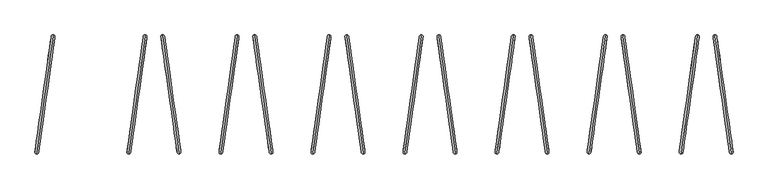
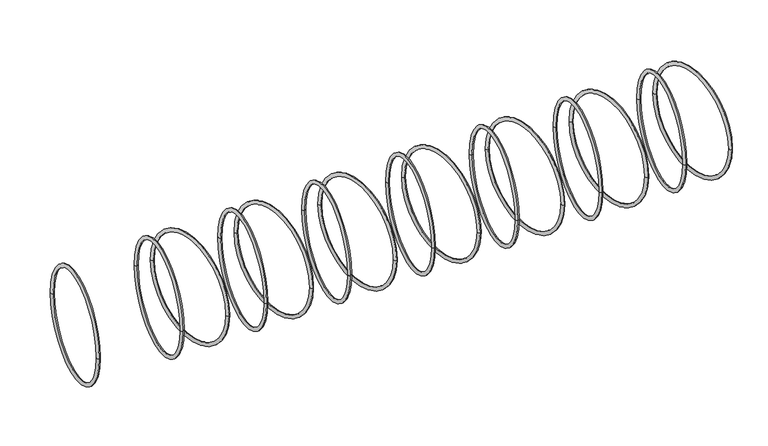
"""IFC4 building model written with IfcOpenShell, lengths in millimetres: geographic element geometry, NLRS_90_SI_WPB_fietsenrek staal_gen_bf : fietsenrek 5500mm 14 plaatsen."""

from ifc_helpers import new_model, si_unit, point, frame, origin, place, context, project, spatial, circle_curve, ellipse_curve, trimmed, source, transform, mapped, element, save
from ifc_brep_helpers import revolved_surface, advanced_brep


def geographic_element_08e1790a(model_context):
    return source(origin(), model_context, "Body", "AdvancedBrep", [
        advanced_brep(
        [(2160.5888305, -21.9255981, 304.7993564), (2092.0982681, -509.2612714, 304.7993564), (2089.8888952, -524.981777, 304.7993564), (2162.7982034, -6.2050925, 304.7993564)],
        [
            (0, 1, circle_curve(frame((2126.3435493, -265.5934347, 304.7993564), z_axis=(0.990268068741571, -0.13917310096006058, 0.0), x_axis=(-0.13917310096006058, -0.990268068741571, 0.0)), 246.0625)),
            (1, 2, circle_curve(frame((2090.9935817, -517.1215242, 304.7993564), z_axis=(0.0, 0.0, 1.0), x_axis=(0.13917310096006055, 0.990268068741571, 0.0)), 7.9375)),
            (2, 3, circle_curve(frame((2126.3435493, -265.5934347, 304.7993564), z_axis=(-0.990268068741571, 0.13917310096006058, 0.0), x_axis=(-0.13917310096006058, -0.990268068741571, 0.0)), 261.9375)),
            (3, 0, circle_curve(frame((2161.6935169, -14.0653453, 304.7993564), z_axis=(0.0, 0.0, 1.0), x_axis=(-0.1391731009600606, -0.990268068741571, 0.0)), 7.9375)),
            (2, 1, circle_curve(frame((2090.9935817, -517.1215242, 304.7993564), z_axis=(0.0, 0.0, 1.0), x_axis=(0.13917310096006055, 0.990268068741571, 0.0)), 7.9375)),
            (0, 3, circle_curve(frame((2161.6935169, -14.0653453, 304.7993564), z_axis=(0.0, 0.0, 1.0), x_axis=(-0.1391731009600606, -0.990268068741571, 0.0)), 7.9375)),
            (1, 0, circle_curve(frame((2126.3435493, -265.5934347, 304.7993564), z_axis=(0.990268068741571, -0.13917310096006058, 0.0), x_axis=(0.13917310096006058, 0.990268068741571, 0.0)), 246.0625)),
            (3, 2, circle_curve(frame((2126.3435493, -265.5934347, 304.7993564), z_axis=(-0.990268068741571, 0.13917310096006058, 0.0), x_axis=(0.13917310096006058, 0.990268068741571, 0.0)), 261.9375)),
        ],
        [
            revolved_surface(trimmed(ellipse_curve(frame((2090.9935817, -517.1215242, 304.7993564), z_axis=(0.0, 0.0, -1.0), x_axis=(0.13917310096006055, 0.990268068741571, 0.0)), 7.9375, 7.9375), [point((2089.8888952, -524.981777, 304.7993564))], [point((2092.0982681, -509.2612714, 304.7993564))], True, "CARTESIAN"), (2314.9896164, -292.1059105, 304.7993564), (-0.990268068741571, 0.13917310096006058, 0.0)),
            revolved_surface(trimmed(ellipse_curve(frame((2090.9935817, -517.1215242, 304.7993564), z_axis=(0.0, 0.0, -1.0), x_axis=(0.13917310096006055, 0.990268068741571, 0.0)), 7.9375, 7.9375), [point((2092.0982681, -509.2612714, 304.7993564))], [point((2089.8888952, -524.981777, 304.7993564))], True, "CARTESIAN"), (2314.9896164, -292.1059105, 304.7993564), (-0.990268068741571, 0.13917310096006058, 0.0)),
            revolved_surface(trimmed(ellipse_curve(frame((2161.6935169, -14.0653453, 304.7993564), z_axis=(0.0, 0.0, 1.0), x_axis=(-0.13917310096006055, -0.990268068741571, 0.0)), 7.9375, 7.9375), [point((2162.7982034, -6.2050925, 304.7993564))], [point((2160.5888305, -21.9255981, 304.7993564))], True, "CARTESIAN"), (2314.9896164, -292.1059105, 304.7993564), (-0.990268068741571, 0.13917310096006058, 0.0)),
            revolved_surface(trimmed(ellipse_curve(frame((2161.6935169, -14.0653453, 304.7993564), z_axis=(0.0, 0.0, 1.0), x_axis=(-0.13917310096006055, -0.990268068741571, 0.0)), 7.9375, 7.9375), [point((2160.5888305, -21.9255981, 304.7993564))], [point((2162.7982034, -6.2050925, 304.7993564))], True, "CARTESIAN"), (2314.9896164, -292.1059105, 304.7993564), (-0.990268068741571, 0.13917310096006058, 0.0)),
        ],
        [
            (0, [[1, 2, 3, 4]]),
            (1, [[-3, 5, -1, 6]]),
            (2, [[7, -4, 8, -2]]),
            (3, [[-8, -6, -7, -5]]),
        ],
    ),
        advanced_brep(
        [(2239.4111695, -21.9255981, 304.7993564), (2307.9017319, -509.2612714, 304.7993564), (2310.1111048, -524.981777, 304.7993564), (2237.2017966, -6.2050925, 304.7993564)],
        [
            (0, 1, circle_curve(frame((2273.6564507, -265.5934347, 304.7993564), z_axis=(0.9902680687415715, 0.1391731009600577, 0.0), x_axis=(0.1391731009600577, -0.9902680687415715, 0.0)), 246.0625)),
            (1, 2, circle_curve(frame((2309.0064183, -517.1215242, 304.7993564), z_axis=(0.0, 0.0, 1.0), x_axis=(-0.13917310096005775, 0.9902680687415715, 0.0)), 7.9375)),
            (2, 3, circle_curve(frame((2273.6564507, -265.5934347, 304.7993564), z_axis=(-0.9902680687415715, -0.1391731009600577, 0.0), x_axis=(0.1391731009600577, -0.9902680687415715, 0.0)), 261.9375)),
            (3, 0, circle_curve(frame((2238.3064831, -14.0653453, 304.7993564), z_axis=(0.0, 0.0, 1.0), x_axis=(0.13917310096005764, -0.9902680687415715, 0.0)), 7.9375)),
            (2, 1, circle_curve(frame((2309.0064183, -517.1215242, 304.7993564), z_axis=(0.0, 0.0, 1.0), x_axis=(-0.13917310096005775, 0.9902680687415715, 0.0)), 7.9375)),
            (0, 3, circle_curve(frame((2238.3064831, -14.0653453, 304.7993564), z_axis=(0.0, 0.0, 1.0), x_axis=(0.13917310096005764, -0.9902680687415715, 0.0)), 7.9375)),
            (1, 0, circle_curve(frame((2273.6564507, -265.5934347, 304.7993564), z_axis=(0.9902680687415715, 0.1391731009600577, 0.0), x_axis=(-0.1391731009600577, 0.9902680687415715, 0.0)), 246.0625)),
            (3, 2, circle_curve(frame((2273.6564507, -265.5934347, 304.7993564), z_axis=(-0.9902680687415715, -0.1391731009600577, 0.0), x_axis=(-0.1391731009600577, 0.9902680687415715, 0.0)), 261.9375)),
        ],
        [
            revolved_surface(trimmed(ellipse_curve(frame((2309.0064183, -517.1215242, 304.7993564), z_axis=(0.0, 0.0, -1.0), x_axis=(-0.13917310096005775, 0.9902680687415715, 0.0)), 7.9375, 7.9375), [point((2310.1111048, -524.981777, 304.7993564))], [point((2307.9017319, -509.2612714, 304.7993564))], True, "CARTESIAN"), (2085.0103836, -292.1059105, 304.7993564), (-0.9902680687415715, -0.1391731009600577, 0.0)),
            revolved_surface(trimmed(ellipse_curve(frame((2309.0064183, -517.1215242, 304.7993564), z_axis=(0.0, 0.0, -1.0), x_axis=(-0.13917310096005775, 0.9902680687415715, 0.0)), 7.9375, 7.9375), [point((2307.9017319, -509.2612714, 304.7993564))], [point((2310.1111048, -524.981777, 304.7993564))], True, "CARTESIAN"), (2085.0103836, -292.1059105, 304.7993564), (-0.9902680687415715, -0.1391731009600577, 0.0)),
            revolved_surface(trimmed(ellipse_curve(frame((2238.3064831, -14.0653453, 304.7993564), z_axis=(0.0, 0.0, 1.0), x_axis=(0.1391731009600577, -0.9902680687415715, 0.0)), 7.9375, 7.9375), [point((2237.2017966, -6.2050925, 304.7993564))], [point((2239.4111695, -21.9255981, 304.7993564))], True, "CARTESIAN"), (2085.0103836, -292.1059105, 304.7993564), (-0.9902680687415715, -0.1391731009600577, 0.0)),
            revolved_surface(trimmed(ellipse_curve(frame((2238.3064831, -14.0653453, 304.7993564), z_axis=(0.0, 0.0, 1.0), x_axis=(0.1391731009600577, -0.9902680687415715, 0.0)), 7.9375, 7.9375), [point((2239.4111695, -21.9255981, 304.7993564))], [point((2237.2017966, -6.2050925, 304.7993564))], True, "CARTESIAN"), (2085.0103836, -292.1059105, 304.7993564), (-0.9902680687415715, -0.1391731009600577, 0.0)),
        ],
        [
            (0, [[1, 2, 3, 4]]),
            (1, [[-3, 5, -1, 6]]),
            (2, [[7, -4, 8, -2]]),
            (3, [[-8, -6, -7, -5]]),
        ],
    ),
        advanced_brep(
        [(1760.5888305, -21.9255981, 304.7993564), (1692.0982681, -509.2612714, 304.7993564), (1689.8888952, -524.981777, 304.7993564), (1762.7982034, -6.2050925, 304.7993564)],
        [
            (0, 1, circle_curve(frame((1726.3435493, -265.5934347, 304.7993564), z_axis=(0.990268068741571, -0.13917310096006058, 0.0), x_axis=(-0.13917310096006058, -0.990268068741571, 0.0)), 246.0625)),
            (1, 2, circle_curve(frame((1690.9935817, -517.1215242, 304.7993564), z_axis=(0.0, 0.0, 1.0), x_axis=(0.13917310096006055, 0.990268068741571, 0.0)), 7.9375)),
            (2, 3, circle_curve(frame((1726.3435493, -265.5934347, 304.7993564), z_axis=(-0.990268068741571, 0.13917310096006058, 0.0), x_axis=(-0.13917310096006058, -0.990268068741571, 0.0)), 261.9375)),
            (3, 0, circle_curve(frame((1761.6935169, -14.0653453, 304.7993564), z_axis=(0.0, 0.0, 1.0), x_axis=(-0.1391731009600606, -0.990268068741571, 0.0)), 7.9375)),
            (2, 1, circle_curve(frame((1690.9935817, -517.1215242, 304.7993564), z_axis=(0.0, 0.0, 1.0), x_axis=(0.13917310096006055, 0.990268068741571, 0.0)), 7.9375)),
            (0, 3, circle_curve(frame((1761.6935169, -14.0653453, 304.7993564), z_axis=(0.0, 0.0, 1.0), x_axis=(-0.1391731009600606, -0.990268068741571, 0.0)), 7.9375)),
            (1, 0, circle_curve(frame((1726.3435493, -265.5934347, 304.7993564), z_axis=(0.990268068741571, -0.13917310096006058, 0.0), x_axis=(0.13917310096006058, 0.990268068741571, 0.0)), 246.0625)),
            (3, 2, circle_curve(frame((1726.3435493, -265.5934347, 304.7993564), z_axis=(-0.990268068741571, 0.13917310096006058, 0.0), x_axis=(0.13917310096006058, 0.990268068741571, 0.0)), 261.9375)),
        ],
        [
            revolved_surface(trimmed(ellipse_curve(frame((1690.9935817, -517.1215242, 304.7993564), z_axis=(0.0, 0.0, -1.0), x_axis=(0.13917310096006055, 0.990268068741571, 0.0)), 7.9375, 7.9375), [point((1689.8888952, -524.981777, 304.7993564))], [point((1692.0982681, -509.2612714, 304.7993564))], True, "CARTESIAN"), (1914.9896164, -292.1059105, 304.7993564), (-0.990268068741571, 0.13917310096006058, 0.0)),
            revolved_surface(trimmed(ellipse_curve(frame((1690.9935817, -517.1215242, 304.7993564), z_axis=(0.0, 0.0, -1.0), x_axis=(0.13917310096006055, 0.990268068741571, 0.0)), 7.9375, 7.9375), [point((1692.0982681, -509.2612714, 304.7993564))], [point((1689.8888952, -524.981777, 304.7993564))], True, "CARTESIAN"), (1914.9896164, -292.1059105, 304.7993564), (-0.990268068741571, 0.13917310096006058, 0.0)),
            revolved_surface(trimmed(ellipse_curve(frame((1761.6935169, -14.0653453, 304.7993564), z_axis=(0.0, 0.0, 1.0), x_axis=(-0.13917310096006055, -0.990268068741571, 0.0)), 7.9375, 7.9375), [point((1762.7982034, -6.2050925, 304.7993564))], [point((1760.5888305, -21.9255981, 304.7993564))], True, "CARTESIAN"), (1914.9896164, -292.1059105, 304.7993564), (-0.990268068741571, 0.13917310096006058, 0.0)),
            revolved_surface(trimmed(ellipse_curve(frame((1761.6935169, -14.0653453, 304.7993564), z_axis=(0.0, 0.0, 1.0), x_axis=(-0.13917310096006055, -0.990268068741571, 0.0)), 7.9375, 7.9375), [point((1760.5888305, -21.9255981, 304.7993564))], [point((1762.7982034, -6.2050925, 304.7993564))], True, "CARTESIAN"), (1914.9896164, -292.1059105, 304.7993564), (-0.990268068741571, 0.13917310096006058, 0.0)),
        ],
        [
            (0, [[1, 2, 3, 4]]),
            (1, [[-3, 5, -1, 6]]),
            (2, [[7, -4, 8, -2]]),
            (3, [[-8, -6, -7, -5]]),
        ],
    ),
        advanced_brep(
        [(1839.4111695, -21.9255981, 304.7993564), (1907.9017319, -509.2612714, 304.7993564), (1910.1111048, -524.981777, 304.7993564), (1837.2017966, -6.2050925, 304.7993564)],
        [
            (0, 1, circle_curve(frame((1873.6564507, -265.5934347, 304.7993564), z_axis=(0.9902680687415715, 0.1391731009600577, 0.0), x_axis=(0.1391731009600577, -0.9902680687415715, 0.0)), 246.0625)),
            (1, 2, circle_curve(frame((1909.0064183, -517.1215242, 304.7993564), z_axis=(0.0, 0.0, 1.0), x_axis=(-0.13917310096005775, 0.9902680687415715, 0.0)), 7.9375)),
            (2, 3, circle_curve(frame((1873.6564507, -265.5934347, 304.7993564), z_axis=(-0.9902680687415715, -0.1391731009600577, 0.0), x_axis=(0.1391731009600577, -0.9902680687415715, 0.0)), 261.9375)),
            (3, 0, circle_curve(frame((1838.3064831, -14.0653453, 304.7993564), z_axis=(0.0, 0.0, 1.0), x_axis=(0.13917310096005764, -0.9902680687415715, 0.0)), 7.9375)),
            (2, 1, circle_curve(frame((1909.0064183, -517.1215242, 304.7993564), z_axis=(0.0, 0.0, 1.0), x_axis=(-0.13917310096005775, 0.9902680687415715, 0.0)), 7.9375)),
            (0, 3, circle_curve(frame((1838.3064831, -14.0653453, 304.7993564), z_axis=(0.0, 0.0, 1.0), x_axis=(0.13917310096005764, -0.9902680687415715, 0.0)), 7.9375)),
            (1, 0, circle_curve(frame((1873.6564507, -265.5934347, 304.7993564), z_axis=(0.9902680687415715, 0.1391731009600577, 0.0), x_axis=(-0.1391731009600577, 0.9902680687415715, 0.0)), 246.0625)),
            (3, 2, circle_curve(frame((1873.6564507, -265.5934347, 304.7993564), z_axis=(-0.9902680687415715, -0.1391731009600577, 0.0), x_axis=(-0.1391731009600577, 0.9902680687415715, 0.0)), 261.9375)),
        ],
        [
            revolved_surface(trimmed(ellipse_curve(frame((1909.0064183, -517.1215242, 304.7993564), z_axis=(0.0, 0.0, -1.0), x_axis=(-0.13917310096005775, 0.9902680687415715, 0.0)), 7.9375, 7.9375), [point((1910.1111048, -524.981777, 304.7993564))], [point((1907.9017319, -509.2612714, 304.7993564))], True, "CARTESIAN"), (1685.0103836, -292.1059105, 304.7993564), (-0.9902680687415715, -0.1391731009600577, 0.0)),
            revolved_surface(trimmed(ellipse_curve(frame((1909.0064183, -517.1215242, 304.7993564), z_axis=(0.0, 0.0, -1.0), x_axis=(-0.13917310096005775, 0.9902680687415715, 0.0)), 7.9375, 7.9375), [point((1907.9017319, -509.2612714, 304.7993564))], [point((1910.1111048, -524.981777, 304.7993564))], True, "CARTESIAN"), (1685.0103836, -292.1059105, 304.7993564), (-0.9902680687415715, -0.1391731009600577, 0.0)),
            revolved_surface(trimmed(ellipse_curve(frame((1838.3064831, -14.0653453, 304.7993564), z_axis=(0.0, 0.0, 1.0), x_axis=(0.1391731009600577, -0.9902680687415715, 0.0)), 7.9375, 7.9375), [point((1837.2017966, -6.2050925, 304.7993564))], [point((1839.4111695, -21.9255981, 304.7993564))], True, "CARTESIAN"), (1685.0103836, -292.1059105, 304.7993564), (-0.9902680687415715, -0.1391731009600577, 0.0)),
            revolved_surface(trimmed(ellipse_curve(frame((1838.3064831, -14.0653453, 304.7993564), z_axis=(0.0, 0.0, 1.0), x_axis=(0.1391731009600577, -0.9902680687415715, 0.0)), 7.9375, 7.9375), [point((1839.4111695, -21.9255981, 304.7993564))], [point((1837.2017966, -6.2050925, 304.7993564))], True, "CARTESIAN"), (1685.0103836, -292.1059105, 304.7993564), (-0.9902680687415715, -0.1391731009600577, 0.0)),
        ],
        [
            (0, [[1, 2, 3, 4]]),
            (1, [[-3, 5, -1, 6]]),
            (2, [[7, -4, 8, -2]]),
            (3, [[-8, -6, -7, -5]]),
        ],
    ),
        advanced_brep(
        [(1360.5888305, -21.9255981, 304.7993564), (1292.0982681, -509.2612714, 304.7993564), (1289.8888952, -524.981777, 304.7993564), (1362.7982034, -6.2050925, 304.7993564)],
        [
            (0, 1, circle_curve(frame((1326.3435493, -265.5934347, 304.7993564), z_axis=(0.990268068741571, -0.13917310096006058, 0.0), x_axis=(-0.13917310096006058, -0.990268068741571, 0.0)), 246.0625)),
            (1, 2, circle_curve(frame((1290.9935817, -517.1215242, 304.7993564), z_axis=(0.0, 0.0, 1.0), x_axis=(0.13917310096006055, 0.990268068741571, 0.0)), 7.9375)),
            (2, 3, circle_curve(frame((1326.3435493, -265.5934347, 304.7993564), z_axis=(-0.990268068741571, 0.13917310096006058, 0.0), x_axis=(-0.13917310096006058, -0.990268068741571, 0.0)), 261.9375)),
            (3, 0, circle_curve(frame((1361.6935169, -14.0653453, 304.7993564), z_axis=(0.0, 0.0, 1.0), x_axis=(-0.1391731009600606, -0.990268068741571, 0.0)), 7.9375)),
            (2, 1, circle_curve(frame((1290.9935817, -517.1215242, 304.7993564), z_axis=(0.0, 0.0, 1.0), x_axis=(0.13917310096006055, 0.990268068741571, 0.0)), 7.9375)),
            (0, 3, circle_curve(frame((1361.6935169, -14.0653453, 304.7993564), z_axis=(0.0, 0.0, 1.0), x_axis=(-0.1391731009600606, -0.990268068741571, 0.0)), 7.9375)),
            (1, 0, circle_curve(frame((1326.3435493, -265.5934347, 304.7993564), z_axis=(0.990268068741571, -0.13917310096006058, 0.0), x_axis=(0.13917310096006058, 0.990268068741571, 0.0)), 246.0625)),
            (3, 2, circle_curve(frame((1326.3435493, -265.5934347, 304.7993564), z_axis=(-0.990268068741571, 0.13917310096006058, 0.0), x_axis=(0.13917310096006058, 0.990268068741571, 0.0)), 261.9375)),
        ],
        [
            revolved_surface(trimmed(ellipse_curve(frame((1290.9935817, -517.1215242, 304.7993564), z_axis=(0.0, 0.0, -1.0), x_axis=(0.13917310096006055, 0.990268068741571, 0.0)), 7.9375, 7.9375), [point((1289.8888952, -524.981777, 304.7993564))], [point((1292.0982681, -509.2612714, 304.7993564))], True, "CARTESIAN"), (1514.9896164, -292.1059105, 304.7993564), (-0.990268068741571, 0.13917310096006058, 0.0)),
            revolved_surface(trimmed(ellipse_curve(frame((1290.9935817, -517.1215242, 304.7993564), z_axis=(0.0, 0.0, -1.0), x_axis=(0.13917310096006055, 0.990268068741571, 0.0)), 7.9375, 7.9375), [point((1292.0982681, -509.2612714, 304.7993564))], [point((1289.8888952, -524.981777, 304.7993564))], True, "CARTESIAN"), (1514.9896164, -292.1059105, 304.7993564), (-0.990268068741571, 0.13917310096006058, 0.0)),
            revolved_surface(trimmed(ellipse_curve(frame((1361.6935169, -14.0653453, 304.7993564), z_axis=(0.0, 0.0, 1.0), x_axis=(-0.13917310096006055, -0.990268068741571, 0.0)), 7.9375, 7.9375), [point((1362.7982034, -6.2050925, 304.7993564))], [point((1360.5888305, -21.9255981, 304.7993564))], True, "CARTESIAN"), (1514.9896164, -292.1059105, 304.7993564), (-0.990268068741571, 0.13917310096006058, 0.0)),
            revolved_surface(trimmed(ellipse_curve(frame((1361.6935169, -14.0653453, 304.7993564), z_axis=(0.0, 0.0, 1.0), x_axis=(-0.13917310096006055, -0.990268068741571, 0.0)), 7.9375, 7.9375), [point((1360.5888305, -21.9255981, 304.7993564))], [point((1362.7982034, -6.2050925, 304.7993564))], True, "CARTESIAN"), (1514.9896164, -292.1059105, 304.7993564), (-0.990268068741571, 0.13917310096006058, 0.0)),
        ],
        [
            (0, [[1, 2, 3, 4]]),
            (1, [[-3, 5, -1, 6]]),
            (2, [[7, -4, 8, -2]]),
            (3, [[-8, -6, -7, -5]]),
        ],
    ),
        advanced_brep(
        [(1439.4111695, -21.9255981, 304.7993564), (1507.9017319, -509.2612714, 304.7993564), (1510.1111048, -524.981777, 304.7993564), (1437.2017966, -6.2050925, 304.7993564)],
        [
            (0, 1, circle_curve(frame((1473.6564507, -265.5934347, 304.7993564), z_axis=(0.9902680687415715, 0.1391731009600577, 0.0), x_axis=(0.1391731009600577, -0.9902680687415715, 0.0)), 246.0625)),
            (1, 2, circle_curve(frame((1509.0064183, -517.1215242, 304.7993564), z_axis=(0.0, 0.0, 1.0), x_axis=(-0.13917310096005775, 0.9902680687415715, 0.0)), 7.9375)),
            (2, 3, circle_curve(frame((1473.6564507, -265.5934347, 304.7993564), z_axis=(-0.9902680687415715, -0.1391731009600577, 0.0), x_axis=(0.1391731009600577, -0.9902680687415715, 0.0)), 261.9375)),
            (3, 0, circle_curve(frame((1438.3064831, -14.0653453, 304.7993564), z_axis=(0.0, 0.0, 1.0), x_axis=(0.13917310096005764, -0.9902680687415715, 0.0)), 7.9375)),
            (2, 1, circle_curve(frame((1509.0064183, -517.1215242, 304.7993564), z_axis=(0.0, 0.0, 1.0), x_axis=(-0.13917310096005775, 0.9902680687415715, 0.0)), 7.9375)),
            (0, 3, circle_curve(frame((1438.3064831, -14.0653453, 304.7993564), z_axis=(0.0, 0.0, 1.0), x_axis=(0.13917310096005764, -0.9902680687415715, 0.0)), 7.9375)),
            (1, 0, circle_curve(frame((1473.6564507, -265.5934347, 304.7993564), z_axis=(0.9902680687415715, 0.1391731009600577, 0.0), x_axis=(-0.1391731009600577, 0.9902680687415715, 0.0)), 246.0625)),
            (3, 2, circle_curve(frame((1473.6564507, -265.5934347, 304.7993564), z_axis=(-0.9902680687415715, -0.1391731009600577, 0.0), x_axis=(-0.1391731009600577, 0.9902680687415715, 0.0)), 261.9375)),
        ],
        [
            revolved_surface(trimmed(ellipse_curve(frame((1509.0064183, -517.1215242, 304.7993564), z_axis=(0.0, 0.0, -1.0), x_axis=(-0.13917310096005775, 0.9902680687415715, 0.0)), 7.9375, 7.9375), [point((1510.1111048, -524.981777, 304.7993564))], [point((1507.9017319, -509.2612714, 304.7993564))], True, "CARTESIAN"), (1285.0103836, -292.1059105, 304.7993564), (-0.9902680687415715, -0.1391731009600577, 0.0)),
            revolved_surface(trimmed(ellipse_curve(frame((1509.0064183, -517.1215242, 304.7993564), z_axis=(0.0, 0.0, -1.0), x_axis=(-0.13917310096005775, 0.9902680687415715, 0.0)), 7.9375, 7.9375), [point((1507.9017319, -509.2612714, 304.7993564))], [point((1510.1111048, -524.981777, 304.7993564))], True, "CARTESIAN"), (1285.0103836, -292.1059105, 304.7993564), (-0.9902680687415715, -0.1391731009600577, 0.0)),
            revolved_surface(trimmed(ellipse_curve(frame((1438.3064831, -14.0653453, 304.7993564), z_axis=(0.0, 0.0, 1.0), x_axis=(0.1391731009600577, -0.9902680687415715, 0.0)), 7.9375, 7.9375), [point((1437.2017966, -6.2050925, 304.7993564))], [point((1439.4111695, -21.9255981, 304.7993564))], True, "CARTESIAN"), (1285.0103836, -292.1059105, 304.7993564), (-0.9902680687415715, -0.1391731009600577, 0.0)),
            revolved_surface(trimmed(ellipse_curve(frame((1438.3064831, -14.0653453, 304.7993564), z_axis=(0.0, 0.0, 1.0), x_axis=(0.1391731009600577, -0.9902680687415715, 0.0)), 7.9375, 7.9375), [point((1439.4111695, -21.9255981, 304.7993564))], [point((1437.2017966, -6.2050925, 304.7993564))], True, "CARTESIAN"), (1285.0103836, -292.1059105, 304.7993564), (-0.9902680687415715, -0.1391731009600577, 0.0)),
        ],
        [
            (0, [[1, 2, 3, 4]]),
            (1, [[-3, 5, -1, 6]]),
            (2, [[7, -4, 8, -2]]),
            (3, [[-8, -6, -7, -5]]),
        ],
    ),
        advanced_brep(
        [(960.5888305, -21.9255981, 304.7993564), (892.0982681, -509.2612714, 304.7993564), (889.8888952, -524.981777, 304.7993564), (962.7982034, -6.2050925, 304.7993564)],
        [
            (0, 1, circle_curve(frame((926.3435493, -265.5934347, 304.7993564), z_axis=(0.990268068741571, -0.13917310096006058, 0.0), x_axis=(-0.13917310096006058, -0.990268068741571, 0.0)), 246.0625)),
            (1, 2, circle_curve(frame((890.9935817, -517.1215242, 304.7993564), z_axis=(0.0, 0.0, 1.0), x_axis=(0.13917310096006055, 0.990268068741571, 0.0)), 7.9375)),
            (2, 3, circle_curve(frame((926.3435493, -265.5934347, 304.7993564), z_axis=(-0.990268068741571, 0.13917310096006058, 0.0), x_axis=(-0.13917310096006058, -0.990268068741571, 0.0)), 261.9375)),
            (3, 0, circle_curve(frame((961.6935169, -14.0653453, 304.7993564), z_axis=(0.0, 0.0, 1.0), x_axis=(-0.1391731009600606, -0.990268068741571, 0.0)), 7.9375)),
            (2, 1, circle_curve(frame((890.9935817, -517.1215242, 304.7993564), z_axis=(0.0, 0.0, 1.0), x_axis=(0.13917310096006055, 0.990268068741571, 0.0)), 7.9375)),
            (0, 3, circle_curve(frame((961.6935169, -14.0653453, 304.7993564), z_axis=(0.0, 0.0, 1.0), x_axis=(-0.1391731009600606, -0.990268068741571, 0.0)), 7.9375)),
            (1, 0, circle_curve(frame((926.3435493, -265.5934347, 304.7993564), z_axis=(0.990268068741571, -0.13917310096006058, 0.0), x_axis=(0.13917310096006058, 0.990268068741571, 0.0)), 246.0625)),
            (3, 2, circle_curve(frame((926.3435493, -265.5934347, 304.7993564), z_axis=(-0.990268068741571, 0.13917310096006058, 0.0), x_axis=(0.13917310096006058, 0.990268068741571, 0.0)), 261.9375)),
        ],
        [
            revolved_surface(trimmed(ellipse_curve(frame((890.9935817, -517.1215242, 304.7993564), z_axis=(0.0, 0.0, -1.0), x_axis=(0.13917310096006055, 0.990268068741571, 0.0)), 7.9375, 7.9375), [point((889.8888952, -524.981777, 304.7993564))], [point((892.0982681, -509.2612714, 304.7993564))], True, "CARTESIAN"), (1114.9896164, -292.1059105, 304.7993564), (-0.990268068741571, 0.13917310096006058, 0.0)),
            revolved_surface(trimmed(ellipse_curve(frame((890.9935817, -517.1215242, 304.7993564), z_axis=(0.0, 0.0, -1.0), x_axis=(0.13917310096006055, 0.990268068741571, 0.0)), 7.9375, 7.9375), [point((892.0982681, -509.2612714, 304.7993564))], [point((889.8888952, -524.981777, 304.7993564))], True, "CARTESIAN"), (1114.9896164, -292.1059105, 304.7993564), (-0.990268068741571, 0.13917310096006058, 0.0)),
            revolved_surface(trimmed(ellipse_curve(frame((961.6935169, -14.0653453, 304.7993564), z_axis=(0.0, 0.0, 1.0), x_axis=(-0.13917310096006055, -0.990268068741571, 0.0)), 7.9375, 7.9375), [point((962.7982034, -6.2050925, 304.7993564))], [point((960.5888305, -21.9255981, 304.7993564))], True, "CARTESIAN"), (1114.9896164, -292.1059105, 304.7993564), (-0.990268068741571, 0.13917310096006058, 0.0)),
            revolved_surface(trimmed(ellipse_curve(frame((961.6935169, -14.0653453, 304.7993564), z_axis=(0.0, 0.0, 1.0), x_axis=(-0.13917310096006055, -0.990268068741571, 0.0)), 7.9375, 7.9375), [point((960.5888305, -21.9255981, 304.7993564))], [point((962.7982034, -6.2050925, 304.7993564))], True, "CARTESIAN"), (1114.9896164, -292.1059105, 304.7993564), (-0.990268068741571, 0.13917310096006058, 0.0)),
        ],
        [
            (0, [[1, 2, 3, 4]]),
            (1, [[-3, 5, -1, 6]]),
            (2, [[7, -4, 8, -2]]),
            (3, [[-8, -6, -7, -5]]),
        ],
    ),
        advanced_brep(
        [(1039.4111695, -21.9255981, 304.7993564), (1107.9017319, -509.2612714, 304.7993564), (1110.1111048, -524.981777, 304.7993564), (1037.2017966, -6.2050925, 304.7993564)],
        [
            (0, 1, circle_curve(frame((1073.6564507, -265.5934347, 304.7993564), z_axis=(0.9902680687415715, 0.1391731009600577, 0.0), x_axis=(0.1391731009600577, -0.9902680687415715, 0.0)), 246.0625)),
            (1, 2, circle_curve(frame((1109.0064183, -517.1215242, 304.7993564), z_axis=(0.0, 0.0, 1.0), x_axis=(-0.13917310096005775, 0.9902680687415715, 0.0)), 7.9375)),
            (2, 3, circle_curve(frame((1073.6564507, -265.5934347, 304.7993564), z_axis=(-0.9902680687415715, -0.1391731009600577, 0.0), x_axis=(0.1391731009600577, -0.9902680687415715, 0.0)), 261.9375)),
            (3, 0, circle_curve(frame((1038.3064831, -14.0653453, 304.7993564), z_axis=(0.0, 0.0, 1.0), x_axis=(0.13917310096005764, -0.9902680687415715, 0.0)), 7.9375)),
            (2, 1, circle_curve(frame((1109.0064183, -517.1215242, 304.7993564), z_axis=(0.0, 0.0, 1.0), x_axis=(-0.13917310096005775, 0.9902680687415715, 0.0)), 7.9375)),
            (0, 3, circle_curve(frame((1038.3064831, -14.0653453, 304.7993564), z_axis=(0.0, 0.0, 1.0), x_axis=(0.13917310096005764, -0.9902680687415715, 0.0)), 7.9375)),
            (1, 0, circle_curve(frame((1073.6564507, -265.5934347, 304.7993564), z_axis=(0.9902680687415715, 0.1391731009600577, 0.0), x_axis=(-0.1391731009600577, 0.9902680687415715, 0.0)), 246.0625)),
            (3, 2, circle_curve(frame((1073.6564507, -265.5934347, 304.7993564), z_axis=(-0.9902680687415715, -0.1391731009600577, 0.0), x_axis=(-0.1391731009600577, 0.9902680687415715, 0.0)), 261.9375)),
        ],
        [
            revolved_surface(trimmed(ellipse_curve(frame((1109.0064183, -517.1215242, 304.7993564), z_axis=(0.0, 0.0, -1.0), x_axis=(-0.13917310096005775, 0.9902680687415715, 0.0)), 7.9375, 7.9375), [point((1110.1111048, -524.981777, 304.7993564))], [point((1107.9017319, -509.2612714, 304.7993564))], True, "CARTESIAN"), (885.0103836, -292.1059105, 304.7993564), (-0.9902680687415715, -0.1391731009600577, 0.0)),
            revolved_surface(trimmed(ellipse_curve(frame((1109.0064183, -517.1215242, 304.7993564), z_axis=(0.0, 0.0, -1.0), x_axis=(-0.13917310096005775, 0.9902680687415715, 0.0)), 7.9375, 7.9375), [point((1107.9017319, -509.2612714, 304.7993564))], [point((1110.1111048, -524.981777, 304.7993564))], True, "CARTESIAN"), (885.0103836, -292.1059105, 304.7993564), (-0.9902680687415715, -0.1391731009600577, 0.0)),
            revolved_surface(trimmed(ellipse_curve(frame((1038.3064831, -14.0653453, 304.7993564), z_axis=(0.0, 0.0, 1.0), x_axis=(0.1391731009600577, -0.9902680687415715, 0.0)), 7.9375, 7.9375), [point((1037.2017966, -6.2050925, 304.7993564))], [point((1039.4111695, -21.9255981, 304.7993564))], True, "CARTESIAN"), (885.0103836, -292.1059105, 304.7993564), (-0.9902680687415715, -0.1391731009600577, 0.0)),
            revolved_surface(trimmed(ellipse_curve(frame((1038.3064831, -14.0653453, 304.7993564), z_axis=(0.0, 0.0, 1.0), x_axis=(0.1391731009600577, -0.9902680687415715, 0.0)), 7.9375, 7.9375), [point((1039.4111695, -21.9255981, 304.7993564))], [point((1037.2017966, -6.2050925, 304.7993564))], True, "CARTESIAN"), (885.0103836, -292.1059105, 304.7993564), (-0.9902680687415715, -0.1391731009600577, 0.0)),
        ],
        [
            (0, [[1, 2, 3, 4]]),
            (1, [[-3, 5, -1, 6]]),
            (2, [[7, -4, 8, -2]]),
            (3, [[-8, -6, -7, -5]]),
        ],
    ),
        advanced_brep(
        [(560.5888305, -21.9255981, 304.7993564), (492.0982681, -509.2612714, 304.7993564), (489.8888952, -524.981777, 304.7993564), (562.7982034, -6.2050925, 304.7993564)],
        [
            (0, 1, circle_curve(frame((526.3435493, -265.5934347, 304.7993564), z_axis=(0.990268068741571, -0.13917310096006058, 0.0), x_axis=(-0.13917310096006058, -0.990268068741571, 0.0)), 246.0625)),
            (1, 2, circle_curve(frame((490.9935817, -517.1215242, 304.7993564), z_axis=(0.0, 0.0, 1.0), x_axis=(0.13917310096006055, 0.990268068741571, 0.0)), 7.9375)),
            (2, 3, circle_curve(frame((526.3435493, -265.5934347, 304.7993564), z_axis=(-0.990268068741571, 0.13917310096006058, 0.0), x_axis=(-0.13917310096006058, -0.990268068741571, 0.0)), 261.9375)),
            (3, 0, circle_curve(frame((561.6935169, -14.0653453, 304.7993564), z_axis=(0.0, 0.0, 1.0), x_axis=(-0.1391731009600606, -0.990268068741571, 0.0)), 7.9375)),
            (2, 1, circle_curve(frame((490.9935817, -517.1215242, 304.7993564), z_axis=(0.0, 0.0, 1.0), x_axis=(0.13917310096006055, 0.990268068741571, 0.0)), 7.9375)),
            (0, 3, circle_curve(frame((561.6935169, -14.0653453, 304.7993564), z_axis=(0.0, 0.0, 1.0), x_axis=(-0.1391731009600606, -0.990268068741571, 0.0)), 7.9375)),
            (1, 0, circle_curve(frame((526.3435493, -265.5934347, 304.7993564), z_axis=(0.990268068741571, -0.13917310096006058, 0.0), x_axis=(0.13917310096006058, 0.990268068741571, 0.0)), 246.0625)),
            (3, 2, circle_curve(frame((526.3435493, -265.5934347, 304.7993564), z_axis=(-0.990268068741571, 0.13917310096006058, 0.0), x_axis=(0.13917310096006058, 0.990268068741571, 0.0)), 261.9375)),
        ],
        [
            revolved_surface(trimmed(ellipse_curve(frame((490.9935817, -517.1215242, 304.7993564), z_axis=(0.0, 0.0, -1.0), x_axis=(0.13917310096006055, 0.990268068741571, 0.0)), 7.9375, 7.9375), [point((489.8888952, -524.981777, 304.7993564))], [point((492.0982681, -509.2612714, 304.7993564))], True, "CARTESIAN"), (714.9896164, -292.1059105, 304.7993564), (-0.990268068741571, 0.13917310096006058, 0.0)),
            revolved_surface(trimmed(ellipse_curve(frame((490.9935817, -517.1215242, 304.7993564), z_axis=(0.0, 0.0, -1.0), x_axis=(0.13917310096006055, 0.990268068741571, 0.0)), 7.9375, 7.9375), [point((492.0982681, -509.2612714, 304.7993564))], [point((489.8888952, -524.981777, 304.7993564))], True, "CARTESIAN"), (714.9896164, -292.1059105, 304.7993564), (-0.990268068741571, 0.13917310096006058, 0.0)),
            revolved_surface(trimmed(ellipse_curve(frame((561.6935169, -14.0653453, 304.7993564), z_axis=(0.0, 0.0, 1.0), x_axis=(-0.13917310096006055, -0.990268068741571, 0.0)), 7.9375, 7.9375), [point((562.7982034, -6.2050925, 304.7993564))], [point((560.5888305, -21.9255981, 304.7993564))], True, "CARTESIAN"), (714.9896164, -292.1059105, 304.7993564), (-0.990268068741571, 0.13917310096006058, 0.0)),
            revolved_surface(trimmed(ellipse_curve(frame((561.6935169, -14.0653453, 304.7993564), z_axis=(0.0, 0.0, 1.0), x_axis=(-0.13917310096006055, -0.990268068741571, 0.0)), 7.9375, 7.9375), [point((560.5888305, -21.9255981, 304.7993564))], [point((562.7982034, -6.2050925, 304.7993564))], True, "CARTESIAN"), (714.9896164, -292.1059105, 304.7993564), (-0.990268068741571, 0.13917310096006058, 0.0)),
        ],
        [
            (0, [[1, 2, 3, 4]]),
            (1, [[-3, 5, -1, 6]]),
            (2, [[7, -4, 8, -2]]),
            (3, [[-8, -6, -7, -5]]),
        ],
    ),
        advanced_brep(
        [(639.4111695, -21.9255981, 304.7993564), (707.9017319, -509.2612714, 304.7993564), (710.1111048, -524.981777, 304.7993564), (637.2017966, -6.2050925, 304.7993564)],
        [
            (0, 1, circle_curve(frame((673.6564507, -265.5934347, 304.7993564), z_axis=(0.9902680687415715, 0.1391731009600577, 0.0), x_axis=(0.1391731009600577, -0.9902680687415715, 0.0)), 246.0625)),
            (1, 2, circle_curve(frame((709.0064183, -517.1215242, 304.7993564), z_axis=(0.0, 0.0, 1.0), x_axis=(-0.13917310096005775, 0.9902680687415715, 0.0)), 7.9375)),
            (2, 3, circle_curve(frame((673.6564507, -265.5934347, 304.7993564), z_axis=(-0.9902680687415715, -0.1391731009600577, 0.0), x_axis=(0.1391731009600577, -0.9902680687415715, 0.0)), 261.9375)),
            (3, 0, circle_curve(frame((638.3064831, -14.0653453, 304.7993564), z_axis=(0.0, 0.0, 1.0), x_axis=(0.13917310096005764, -0.9902680687415715, 0.0)), 7.9375)),
            (2, 1, circle_curve(frame((709.0064183, -517.1215242, 304.7993564), z_axis=(0.0, 0.0, 1.0), x_axis=(-0.13917310096005775, 0.9902680687415715, 0.0)), 7.9375)),
            (0, 3, circle_curve(frame((638.3064831, -14.0653453, 304.7993564), z_axis=(0.0, 0.0, 1.0), x_axis=(0.13917310096005764, -0.9902680687415715, 0.0)), 7.9375)),
            (1, 0, circle_curve(frame((673.6564507, -265.5934347, 304.7993564), z_axis=(0.9902680687415715, 0.1391731009600577, 0.0), x_axis=(-0.1391731009600577, 0.9902680687415715, 0.0)), 246.0625)),
            (3, 2, circle_curve(frame((673.6564507, -265.5934347, 304.7993564), z_axis=(-0.9902680687415715, -0.1391731009600577, 0.0), x_axis=(-0.1391731009600577, 0.9902680687415715, 0.0)), 261.9375)),
        ],
        [
            revolved_surface(trimmed(ellipse_curve(frame((709.0064183, -517.1215242, 304.7993564), z_axis=(0.0, 0.0, -1.0), x_axis=(-0.13917310096005775, 0.9902680687415715, 0.0)), 7.9375, 7.9375), [point((710.1111048, -524.981777, 304.7993564))], [point((707.9017319, -509.2612714, 304.7993564))], True, "CARTESIAN"), (485.0103836, -292.1059105, 304.7993564), (-0.9902680687415715, -0.1391731009600577, 0.0)),
            revolved_surface(trimmed(ellipse_curve(frame((709.0064183, -517.1215242, 304.7993564), z_axis=(0.0, 0.0, -1.0), x_axis=(-0.13917310096005775, 0.9902680687415715, 0.0)), 7.9375, 7.9375), [point((707.9017319, -509.2612714, 304.7993564))], [point((710.1111048, -524.981777, 304.7993564))], True, "CARTESIAN"), (485.0103836, -292.1059105, 304.7993564), (-0.9902680687415715, -0.1391731009600577, 0.0)),
            revolved_surface(trimmed(ellipse_curve(frame((638.3064831, -14.0653453, 304.7993564), z_axis=(0.0, 0.0, 1.0), x_axis=(0.1391731009600577, -0.9902680687415715, 0.0)), 7.9375, 7.9375), [point((637.2017966, -6.2050925, 304.7993564))], [point((639.4111695, -21.9255981, 304.7993564))], True, "CARTESIAN"), (485.0103836, -292.1059105, 304.7993564), (-0.9902680687415715, -0.1391731009600577, 0.0)),
            revolved_surface(trimmed(ellipse_curve(frame((638.3064831, -14.0653453, 304.7993564), z_axis=(0.0, 0.0, 1.0), x_axis=(0.1391731009600577, -0.9902680687415715, 0.0)), 7.9375, 7.9375), [point((639.4111695, -21.9255981, 304.7993564))], [point((637.2017966, -6.2050925, 304.7993564))], True, "CARTESIAN"), (485.0103836, -292.1059105, 304.7993564), (-0.9902680687415715, -0.1391731009600577, 0.0)),
        ],
        [
            (0, [[1, 2, 3, 4]]),
            (1, [[-3, 5, -1, 6]]),
            (2, [[7, -4, 8, -2]]),
            (3, [[-8, -6, -7, -5]]),
        ],
    ),
        advanced_brep(
        [(160.5888305, -21.9255981, 304.7993564), (92.0982681, -509.2612714, 304.7993564), (89.8888952, -524.981777, 304.7993564), (162.7982034, -6.2050925, 304.7993564)],
        [
            (0, 1, circle_curve(frame((126.3435493, -265.5934347, 304.7993564), z_axis=(0.990268068741571, -0.13917310096006058, 0.0), x_axis=(-0.13917310096006058, -0.990268068741571, 0.0)), 246.0625)),
            (1, 2, circle_curve(frame((90.9935817, -517.1215242, 304.7993564), z_axis=(0.0, 0.0, 1.0), x_axis=(0.13917310096006055, 0.990268068741571, 0.0)), 7.9375)),
            (2, 3, circle_curve(frame((126.3435493, -265.5934347, 304.7993564), z_axis=(-0.990268068741571, 0.13917310096006058, 0.0), x_axis=(-0.13917310096006058, -0.990268068741571, 0.0)), 261.9375)),
            (3, 0, circle_curve(frame((161.6935169, -14.0653453, 304.7993564), z_axis=(0.0, 0.0, 1.0), x_axis=(-0.1391731009600606, -0.990268068741571, 0.0)), 7.9375)),
            (2, 1, circle_curve(frame((90.9935817, -517.1215242, 304.7993564), z_axis=(0.0, 0.0, 1.0), x_axis=(0.13917310096006055, 0.990268068741571, 0.0)), 7.9375)),
            (0, 3, circle_curve(frame((161.6935169, -14.0653453, 304.7993564), z_axis=(0.0, 0.0, 1.0), x_axis=(-0.1391731009600606, -0.990268068741571, 0.0)), 7.9375)),
            (1, 0, circle_curve(frame((126.3435493, -265.5934347, 304.7993564), z_axis=(0.990268068741571, -0.13917310096006058, 0.0), x_axis=(0.13917310096006058, 0.990268068741571, 0.0)), 246.0625)),
            (3, 2, circle_curve(frame((126.3435493, -265.5934347, 304.7993564), z_axis=(-0.990268068741571, 0.13917310096006058, 0.0), x_axis=(0.13917310096006058, 0.990268068741571, 0.0)), 261.9375)),
        ],
        [
            revolved_surface(trimmed(ellipse_curve(frame((90.9935817, -517.1215242, 304.7993564), z_axis=(0.0, 0.0, -1.0), x_axis=(0.13917310096006055, 0.990268068741571, 0.0)), 7.9375, 7.9375), [point((89.8888952, -524.981777, 304.7993564))], [point((92.0982681, -509.2612714, 304.7993564))], True, "CARTESIAN"), (314.9896164, -292.1059105, 304.7993564), (-0.990268068741571, 0.13917310096006058, 0.0)),
            revolved_surface(trimmed(ellipse_curve(frame((90.9935817, -517.1215242, 304.7993564), z_axis=(0.0, 0.0, -1.0), x_axis=(0.13917310096006055, 0.990268068741571, 0.0)), 7.9375, 7.9375), [point((92.0982681, -509.2612714, 304.7993564))], [point((89.8888952, -524.981777, 304.7993564))], True, "CARTESIAN"), (314.9896164, -292.1059105, 304.7993564), (-0.990268068741571, 0.13917310096006058, 0.0)),
            revolved_surface(trimmed(ellipse_curve(frame((161.6935169, -14.0653453, 304.7993564), z_axis=(0.0, 0.0, 1.0), x_axis=(-0.13917310096006055, -0.990268068741571, 0.0)), 7.9375, 7.9375), [point((162.7982034, -6.2050925, 304.7993564))], [point((160.5888305, -21.9255981, 304.7993564))], True, "CARTESIAN"), (314.9896164, -292.1059105, 304.7993564), (-0.990268068741571, 0.13917310096006058, 0.0)),
            revolved_surface(trimmed(ellipse_curve(frame((161.6935169, -14.0653453, 304.7993564), z_axis=(0.0, 0.0, 1.0), x_axis=(-0.13917310096006055, -0.990268068741571, 0.0)), 7.9375, 7.9375), [point((160.5888305, -21.9255981, 304.7993564))], [point((162.7982034, -6.2050925, 304.7993564))], True, "CARTESIAN"), (314.9896164, -292.1059105, 304.7993564), (-0.990268068741571, 0.13917310096006058, 0.0)),
        ],
        [
            (0, [[1, 2, 3, 4]]),
            (1, [[-3, 5, -1, 6]]),
            (2, [[7, -4, 8, -2]]),
            (3, [[-8, -6, -7, -5]]),
        ],
    ),
        advanced_brep(
        [(239.4111695, -21.9255981, 304.7993564), (307.9017319, -509.2612714, 304.7993564), (310.1111048, -524.981777, 304.7993564), (237.2017966, -6.2050925, 304.7993564)],
        [
            (0, 1, circle_curve(frame((273.6564507, -265.5934347, 304.7993564), z_axis=(0.9902680687415715, 0.1391731009600577, 0.0), x_axis=(0.1391731009600577, -0.9902680687415715, 0.0)), 246.0625)),
            (1, 2, circle_curve(frame((309.0064183, -517.1215242, 304.7993564), z_axis=(0.0, 0.0, 1.0), x_axis=(-0.13917310096005775, 0.9902680687415715, 0.0)), 7.9375)),
            (2, 3, circle_curve(frame((273.6564507, -265.5934347, 304.7993564), z_axis=(-0.9902680687415715, -0.1391731009600577, 0.0), x_axis=(0.1391731009600577, -0.9902680687415715, 0.0)), 261.9375)),
            (3, 0, circle_curve(frame((238.3064831, -14.0653453, 304.7993564), z_axis=(0.0, 0.0, 1.0), x_axis=(0.13917310096005764, -0.9902680687415715, 0.0)), 7.9375)),
            (2, 1, circle_curve(frame((309.0064183, -517.1215242, 304.7993564), z_axis=(0.0, 0.0, 1.0), x_axis=(-0.13917310096005775, 0.9902680687415715, 0.0)), 7.9375)),
            (0, 3, circle_curve(frame((238.3064831, -14.0653453, 304.7993564), z_axis=(0.0, 0.0, 1.0), x_axis=(0.13917310096005764, -0.9902680687415715, 0.0)), 7.9375)),
            (1, 0, circle_curve(frame((273.6564507, -265.5934347, 304.7993564), z_axis=(0.9902680687415715, 0.1391731009600577, 0.0), x_axis=(-0.1391731009600577, 0.9902680687415715, 0.0)), 246.0625)),
            (3, 2, circle_curve(frame((273.6564507, -265.5934347, 304.7993564), z_axis=(-0.9902680687415715, -0.1391731009600577, 0.0), x_axis=(-0.1391731009600577, 0.9902680687415715, 0.0)), 261.9375)),
        ],
        [
            revolved_surface(trimmed(ellipse_curve(frame((309.0064183, -517.1215242, 304.7993564), z_axis=(0.0, 0.0, -1.0), x_axis=(-0.13917310096005775, 0.9902680687415715, 0.0)), 7.9375, 7.9375), [point((310.1111048, -524.981777, 304.7993564))], [point((307.9017319, -509.2612714, 304.7993564))], True, "CARTESIAN"), (85.0103836, -292.1059105, 304.7993564), (-0.9902680687415715, -0.1391731009600577, 0.0)),
            revolved_surface(trimmed(ellipse_curve(frame((309.0064183, -517.1215242, 304.7993564), z_axis=(0.0, 0.0, -1.0), x_axis=(-0.13917310096005775, 0.9902680687415715, 0.0)), 7.9375, 7.9375), [point((307.9017319, -509.2612714, 304.7993564))], [point((310.1111048, -524.981777, 304.7993564))], True, "CARTESIAN"), (85.0103836, -292.1059105, 304.7993564), (-0.9902680687415715, -0.1391731009600577, 0.0)),
            revolved_surface(trimmed(ellipse_curve(frame((238.3064831, -14.0653453, 304.7993564), z_axis=(0.0, 0.0, 1.0), x_axis=(0.1391731009600577, -0.9902680687415715, 0.0)), 7.9375, 7.9375), [point((237.2017966, -6.2050925, 304.7993564))], [point((239.4111695, -21.9255981, 304.7993564))], True, "CARTESIAN"), (85.0103836, -292.1059105, 304.7993564), (-0.9902680687415715, -0.1391731009600577, 0.0)),
            revolved_surface(trimmed(ellipse_curve(frame((238.3064831, -14.0653453, 304.7993564), z_axis=(0.0, 0.0, 1.0), x_axis=(0.1391731009600577, -0.9902680687415715, 0.0)), 7.9375, 7.9375), [point((239.4111695, -21.9255981, 304.7993564))], [point((237.2017966, -6.2050925, 304.7993564))], True, "CARTESIAN"), (85.0103836, -292.1059105, 304.7993564), (-0.9902680687415715, -0.1391731009600577, 0.0)),
        ],
        [
            (0, [[1, 2, 3, 4]]),
            (1, [[-3, 5, -1, 6]]),
            (2, [[7, -4, 8, -2]]),
            (3, [[-8, -6, -7, -5]]),
        ],
    ),
        advanced_brep(
        [(-239.4111695, -21.9255981, 304.7993564), (-307.9017319, -509.2612714, 304.7993564), (-310.1111048, -524.981777, 304.7993564), (-237.2017966, -6.2050925, 304.7993564)],
        [
            (0, 1, circle_curve(frame((-273.6564507, -265.5934347, 304.7993564), z_axis=(0.990268068741571, -0.13917310096006058, 0.0), x_axis=(-0.13917310096006058, -0.990268068741571, 0.0)), 246.0625)),
            (1, 2, circle_curve(frame((-309.0064183, -517.1215242, 304.7993564), z_axis=(0.0, 0.0, 1.0), x_axis=(0.13917310096006055, 0.990268068741571, 0.0)), 7.9375)),
            (2, 3, circle_curve(frame((-273.6564507, -265.5934347, 304.7993564), z_axis=(-0.990268068741571, 0.13917310096006058, 0.0), x_axis=(-0.13917310096006058, -0.990268068741571, 0.0)), 261.9375)),
            (3, 0, circle_curve(frame((-238.3064831, -14.0653453, 304.7993564), z_axis=(0.0, 0.0, 1.0), x_axis=(-0.1391731009600606, -0.990268068741571, 0.0)), 7.9375)),
            (2, 1, circle_curve(frame((-309.0064183, -517.1215242, 304.7993564), z_axis=(0.0, 0.0, 1.0), x_axis=(0.13917310096006055, 0.990268068741571, 0.0)), 7.9375)),
            (0, 3, circle_curve(frame((-238.3064831, -14.0653453, 304.7993564), z_axis=(0.0, 0.0, 1.0), x_axis=(-0.1391731009600606, -0.990268068741571, 0.0)), 7.9375)),
            (1, 0, circle_curve(frame((-273.6564507, -265.5934347, 304.7993564), z_axis=(0.990268068741571, -0.13917310096006058, 0.0), x_axis=(0.13917310096006058, 0.990268068741571, 0.0)), 246.0625)),
            (3, 2, circle_curve(frame((-273.6564507, -265.5934347, 304.7993564), z_axis=(-0.990268068741571, 0.13917310096006058, 0.0), x_axis=(0.13917310096006058, 0.990268068741571, 0.0)), 261.9375)),
        ],
        [
            revolved_surface(trimmed(ellipse_curve(frame((-309.0064183, -517.1215242, 304.7993564), z_axis=(0.0, 0.0, -1.0), x_axis=(0.13917310096006055, 0.990268068741571, 0.0)), 7.9375, 7.9375), [point((-310.1111048, -524.981777, 304.7993564))], [point((-307.9017319, -509.2612714, 304.7993564))], True, "CARTESIAN"), (-85.0103836, -292.1059105, 304.7993564), (-0.990268068741571, 0.13917310096006058, 0.0)),
            revolved_surface(trimmed(ellipse_curve(frame((-309.0064183, -517.1215242, 304.7993564), z_axis=(0.0, 0.0, -1.0), x_axis=(0.13917310096006055, 0.990268068741571, 0.0)), 7.9375, 7.9375), [point((-307.9017319, -509.2612714, 304.7993564))], [point((-310.1111048, -524.981777, 304.7993564))], True, "CARTESIAN"), (-85.0103836, -292.1059105, 304.7993564), (-0.990268068741571, 0.13917310096006058, 0.0)),
            revolved_surface(trimmed(ellipse_curve(frame((-238.3064831, -14.0653453, 304.7993564), z_axis=(0.0, 0.0, 1.0), x_axis=(-0.13917310096006055, -0.990268068741571, 0.0)), 7.9375, 7.9375), [point((-237.2017966, -6.2050925, 304.7993564))], [point((-239.4111695, -21.9255981, 304.7993564))], True, "CARTESIAN"), (-85.0103836, -292.1059105, 304.7993564), (-0.990268068741571, 0.13917310096006058, 0.0)),
            revolved_surface(trimmed(ellipse_curve(frame((-238.3064831, -14.0653453, 304.7993564), z_axis=(0.0, 0.0, 1.0), x_axis=(-0.13917310096006055, -0.990268068741571, 0.0)), 7.9375, 7.9375), [point((-239.4111695, -21.9255981, 304.7993564))], [point((-237.2017966, -6.2050925, 304.7993564))], True, "CARTESIAN"), (-85.0103836, -292.1059105, 304.7993564), (-0.990268068741571, 0.13917310096006058, 0.0)),
        ],
        [
            (0, [[1, 2, 3, 4]]),
            (1, [[-3, 5, -1, 6]]),
            (2, [[7, -4, 8, -2]]),
            (3, [[-8, -6, -7, -5]]),
        ],
    ),
        advanced_brep(
        [(-160.5888305, -21.9255981, 304.7993564), (-92.0982681, -509.2612714, 304.7993564), (-89.8888952, -524.981777, 304.7993564), (-162.7982034, -6.2050925, 304.7993564)],
        [
            (0, 1, circle_curve(frame((-126.3435493, -265.5934347, 304.7993564), z_axis=(0.9902680687415715, 0.1391731009600577, 0.0), x_axis=(0.1391731009600577, -0.9902680687415715, 0.0)), 246.0625)),
            (1, 2, circle_curve(frame((-90.9935817, -517.1215242, 304.7993564), z_axis=(0.0, 0.0, 1.0), x_axis=(-0.13917310096005775, 0.9902680687415715, 0.0)), 7.9375)),
            (2, 3, circle_curve(frame((-126.3435493, -265.5934347, 304.7993564), z_axis=(-0.9902680687415715, -0.1391731009600577, 0.0), x_axis=(0.1391731009600577, -0.9902680687415715, 0.0)), 261.9375)),
            (3, 0, circle_curve(frame((-161.6935169, -14.0653453, 304.7993564), z_axis=(0.0, 0.0, 1.0), x_axis=(0.13917310096005764, -0.9902680687415715, 0.0)), 7.9375)),
            (2, 1, circle_curve(frame((-90.9935817, -517.1215242, 304.7993564), z_axis=(0.0, 0.0, 1.0), x_axis=(-0.13917310096005775, 0.9902680687415715, 0.0)), 7.9375)),
            (0, 3, circle_curve(frame((-161.6935169, -14.0653453, 304.7993564), z_axis=(0.0, 0.0, 1.0), x_axis=(0.13917310096005764, -0.9902680687415715, 0.0)), 7.9375)),
            (1, 0, circle_curve(frame((-126.3435493, -265.5934347, 304.7993564), z_axis=(0.9902680687415715, 0.1391731009600577, 0.0), x_axis=(-0.1391731009600577, 0.9902680687415715, 0.0)), 246.0625)),
            (3, 2, circle_curve(frame((-126.3435493, -265.5934347, 304.7993564), z_axis=(-0.9902680687415715, -0.1391731009600577, 0.0), x_axis=(-0.1391731009600577, 0.9902680687415715, 0.0)), 261.9375)),
        ],
        [
            revolved_surface(trimmed(ellipse_curve(frame((-90.9935817, -517.1215242, 304.7993564), z_axis=(0.0, 0.0, -1.0), x_axis=(-0.13917310096005775, 0.9902680687415715, 0.0)), 7.9375, 7.9375), [point((-89.8888952, -524.981777, 304.7993564))], [point((-92.0982681, -509.2612714, 304.7993564))], True, "CARTESIAN"), (-314.9896164, -292.1059105, 304.7993564), (-0.9902680687415715, -0.1391731009600577, 0.0)),
            revolved_surface(trimmed(ellipse_curve(frame((-90.9935817, -517.1215242, 304.7993564), z_axis=(0.0, 0.0, -1.0), x_axis=(-0.13917310096005775, 0.9902680687415715, 0.0)), 7.9375, 7.9375), [point((-92.0982681, -509.2612714, 304.7993564))], [point((-89.8888952, -524.981777, 304.7993564))], True, "CARTESIAN"), (-314.9896164, -292.1059105, 304.7993564), (-0.9902680687415715, -0.1391731009600577, 0.0)),
            revolved_surface(trimmed(ellipse_curve(frame((-161.6935169, -14.0653453, 304.7993564), z_axis=(0.0, 0.0, 1.0), x_axis=(0.1391731009600577, -0.9902680687415715, 0.0)), 7.9375, 7.9375), [point((-162.7982034, -6.2050925, 304.7993564))], [point((-160.5888305, -21.9255981, 304.7993564))], True, "CARTESIAN"), (-314.9896164, -292.1059105, 304.7993564), (-0.9902680687415715, -0.1391731009600577, 0.0)),
            revolved_surface(trimmed(ellipse_curve(frame((-161.6935169, -14.0653453, 304.7993564), z_axis=(0.0, 0.0, 1.0), x_axis=(0.1391731009600577, -0.9902680687415715, 0.0)), 7.9375, 7.9375), [point((-160.5888305, -21.9255981, 304.7993564))], [point((-162.7982034, -6.2050925, 304.7993564))], True, "CARTESIAN"), (-314.9896164, -292.1059105, 304.7993564), (-0.9902680687415715, -0.1391731009600577, 0.0)),
        ],
        [
            (0, [[1, 2, 3, 4]]),
            (1, [[-3, 5, -1, 6]]),
            (2, [[7, -4, 8, -2]]),
            (3, [[-8, -6, -7, -5]]),
        ],
    ),
        advanced_brep(
        [(-639.4111695, -21.9255981, 304.7993564), (-707.9017319, -509.2612714, 304.7993564), (-710.1111048, -524.981777, 304.7993564), (-637.2017966, -6.2050925, 304.7993564)],
        [
            (0, 1, circle_curve(frame((-673.6564507, -265.5934347, 304.7993564), z_axis=(0.990268068741571, -0.13917310096006058, 0.0), x_axis=(-0.13917310096006058, -0.990268068741571, 0.0)), 246.0625)),
            (1, 2, circle_curve(frame((-709.0064183, -517.1215242, 304.7993564), z_axis=(0.0, 0.0, 1.0), x_axis=(0.13917310096006055, 0.990268068741571, 0.0)), 7.9375)),
            (2, 3, circle_curve(frame((-673.6564507, -265.5934347, 304.7993564), z_axis=(-0.990268068741571, 0.13917310096006058, 0.0), x_axis=(-0.13917310096006058, -0.990268068741571, 0.0)), 261.9375)),
            (3, 0, circle_curve(frame((-638.3064831, -14.0653453, 304.7993564), z_axis=(0.0, 0.0, 1.0), x_axis=(-0.1391731009600606, -0.990268068741571, 0.0)), 7.9375)),
            (2, 1, circle_curve(frame((-709.0064183, -517.1215242, 304.7993564), z_axis=(0.0, 0.0, 1.0), x_axis=(0.13917310096006055, 0.990268068741571, 0.0)), 7.9375)),
            (0, 3, circle_curve(frame((-638.3064831, -14.0653453, 304.7993564), z_axis=(0.0, 0.0, 1.0), x_axis=(-0.1391731009600606, -0.990268068741571, 0.0)), 7.9375)),
            (1, 0, circle_curve(frame((-673.6564507, -265.5934347, 304.7993564), z_axis=(0.990268068741571, -0.13917310096006058, 0.0), x_axis=(0.13917310096006058, 0.990268068741571, 0.0)), 246.0625)),
            (3, 2, circle_curve(frame((-673.6564507, -265.5934347, 304.7993564), z_axis=(-0.990268068741571, 0.13917310096006058, 0.0), x_axis=(0.13917310096006058, 0.990268068741571, 0.0)), 261.9375)),
        ],
        [
            revolved_surface(trimmed(ellipse_curve(frame((-709.0064183, -517.1215242, 304.7993564), z_axis=(0.0, 0.0, -1.0), x_axis=(0.13917310096006055, 0.990268068741571, 0.0)), 7.9375, 7.9375), [point((-710.1111048, -524.981777, 304.7993564))], [point((-707.9017319, -509.2612714, 304.7993564))], True, "CARTESIAN"), (-485.0103836, -292.1059105, 304.7993564), (-0.990268068741571, 0.13917310096006058, 0.0)),
            revolved_surface(trimmed(ellipse_curve(frame((-709.0064183, -517.1215242, 304.7993564), z_axis=(0.0, 0.0, -1.0), x_axis=(0.13917310096006055, 0.990268068741571, 0.0)), 7.9375, 7.9375), [point((-707.9017319, -509.2612714, 304.7993564))], [point((-710.1111048, -524.981777, 304.7993564))], True, "CARTESIAN"), (-485.0103836, -292.1059105, 304.7993564), (-0.990268068741571, 0.13917310096006058, 0.0)),
            revolved_surface(trimmed(ellipse_curve(frame((-638.3064831, -14.0653453, 304.7993564), z_axis=(0.0, 0.0, 1.0), x_axis=(-0.13917310096006055, -0.990268068741571, 0.0)), 7.9375, 7.9375), [point((-637.2017966, -6.2050925, 304.7993564))], [point((-639.4111695, -21.9255981, 304.7993564))], True, "CARTESIAN"), (-485.0103836, -292.1059105, 304.7993564), (-0.990268068741571, 0.13917310096006058, 0.0)),
            revolved_surface(trimmed(ellipse_curve(frame((-638.3064831, -14.0653453, 304.7993564), z_axis=(0.0, 0.0, 1.0), x_axis=(-0.13917310096006055, -0.990268068741571, 0.0)), 7.9375, 7.9375), [point((-639.4111695, -21.9255981, 304.7993564))], [point((-637.2017966, -6.2050925, 304.7993564))], True, "CARTESIAN"), (-485.0103836, -292.1059105, 304.7993564), (-0.990268068741571, 0.13917310096006058, 0.0)),
        ],
        [
            (0, [[1, 2, 3, 4]]),
            (1, [[-3, 5, -1, 6]]),
            (2, [[7, -4, 8, -2]]),
            (3, [[-8, -6, -7, -5]]),
        ],
    ),
    ])


if __name__ == "__main__":
    model = new_model("IFC4")
    model_context = context("Model", 3, world=origin())
    ifc_project = project(units=[si_unit("LENGTHUNIT", "METRE", prefix="MILLI")], contexts=[model_context])
    site = spatial("IfcSite", under=ifc_project)
    building = spatial("IfcBuilding", under=site)
    placement = place(None, origin())
    geographic_element_shape = geographic_element_08e1790a(model_context)
    element("IfcGeographicElement", 1, ObjectType="NLRS_90_SI_WPB_fietsenrek staal_gen_bf : fietsenrek 5500mm 14 plaatsen", at=placement, inside=building, context=model_context, shape_type="MappedRepresentation", body=[
        mapped(geographic_element_shape, transform((0.0, 0.0, 0.0), x_axis=(1.0, 0.0, 0.0), y_axis=(0.0, 1.0, 0.0), z_axis=(0.0, 0.0, 1.0))),
    ])
    save(model, "model.ifc")

# Revit data of these elements
# Type "NLRS_90_SI_WPB_fietsenrek staal_gen_bf : fietsenrek 5500mm 14 plaatsen"
#   Type IFC Predefined Type = "USERDEFINED"
#   Export Type to IFC As = "IfcGeographicElementType"
#   Type IfcGUID = "1jnPA0m7n0IPwpoVFqyx6D"
#   Assembly Code = "90.81"
#   IfcName[Type] = "fietsenrek 5500mm 14 plaatsen"
#   IfcDescription[Type] = "fietsenrek 6m lengte 2x15 plaatsen"
#   IfcObjectType[Type] = "BICYCLE_RACK"
#   IfcExportAs[Type] = "IfcGeographicElementType"
#   IfcExportType[Type] = "USERDEFINED"
#   Model = "generiek"
#   Manufacturer = "generiek"
#   Description = "fietsenrek 6m lengte 2x15 plaatsen"
#   NLRS_C_lengte = 5500.00 mm
#   NLRS_C_afstand = 4000.00 mm
#   rek_dubbel = no
#   NLRS_C_aantal = 14
#   NLRS_C_materiaal = none
#   Default Elevation = 0
